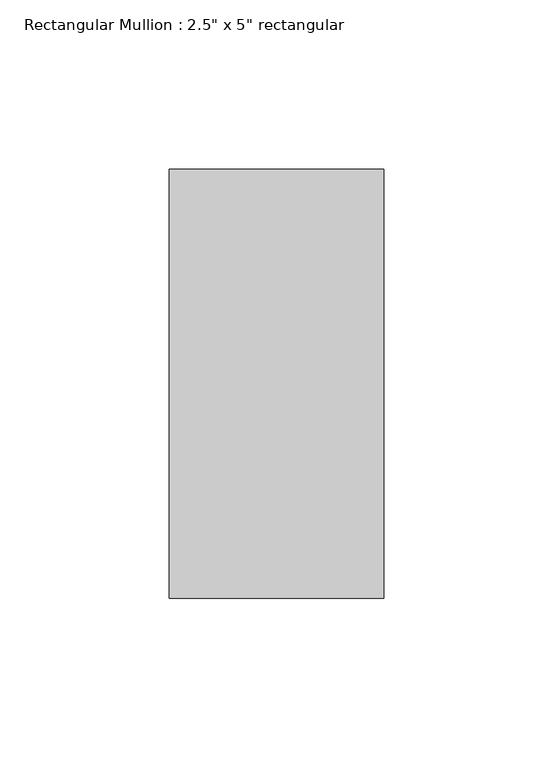
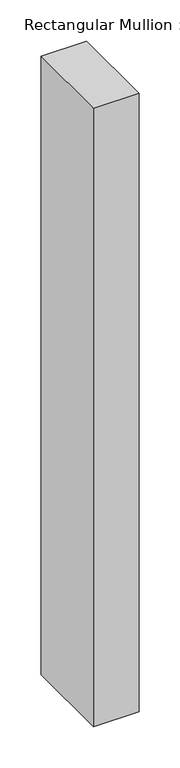
"""IFC4 building model written with IfcOpenShell, lengths in millimetres: member geometry."""

import ifcopenshell
import ifcopenshell.guid

model = None  # the IFC model being written
_history = None  # IfcOwnerHistory: only IFC2X3 demands one
_inside = {}  # id of a spatial element -> (the spatial element, [elements in it])
_under = {}  # id of a project, library or spatial element -> (it, [spatial elements below it])
_declared = {}  # id of a project -> (the project, [libraries it declares])
_typed = {}  # id of a type object -> (the type object, [elements of that type])
_made_of = {}  # id of a material, layer set ... -> (it, [elements and type objects made of it])


def new_model(schema):
    """Start an empty IFC model of exactly this schema.

    Asked for "IFC4X3", IfcOpenShell would pick the latest addendum, in which some entities
    have other attributes; the version numbers below select the first issue.
    IFC2X3 requires an IfcOwnerHistory on every rooted entity: one is made here for all.
    """
    global model, _history
    if schema == "IFC4X3":
        model = ifcopenshell.file(schema_version=(4, 3, 0, 0))
    else:
        model = ifcopenshell.file(schema=schema)
    _inside.clear()
    _under.clear()
    _declared.clear()
    _typed.clear()
    _made_of.clear()
    _history = None
    if model.schema == "IFC2X3":
        org = make("IfcOrganization", Name="unknown")
        user = make(
            "IfcPersonAndOrganization",
            ThePerson=make("IfcPerson", FamilyName="unknown"),
            TheOrganization=org,
        )
        app = make(
            "IfcApplication",
            ApplicationDeveloper=org,
            Version="unknown",
            ApplicationFullName="unknown",
            ApplicationIdentifier="unknown",
        )
        _history = make(
            "IfcOwnerHistory",
            OwningUser=user,
            OwningApplication=app,
            ChangeAction="ADDED",
            CreationDate=0,
        )
    return model


def make(cls, **values):
    """One entity of the class cls with the attributes given. An attribute that is None is left unset."""
    return model.create_entity(
        cls, **{name: value for name, value in values.items() if value is not None}
    )


def rooted(cls, **values):
    """An entity with a GlobalId (a new one), such as an element, a storey or a relation."""
    return make(cls, GlobalId=ifcopenshell.guid.new(), OwnerHistory=_history, **values)


def si_unit(unit_type, name, prefix=None):
    """IfcSIUnit, for example si_unit("LENGTHUNIT", "METRE", prefix="MILLI")."""
    return make("IfcSIUnit", UnitType=unit_type, Prefix=prefix, Name=name)


def assignment(units):
    """IfcUnitAssignment: the units of a project."""
    return None if units is None else make("IfcUnitAssignment", Units=units)


def point(xyz):
    """IfcCartesianPoint."""
    return None if xyz is None else make("IfcCartesianPoint", Coordinates=xyz)


def direction(xyz):
    """IfcDirection."""
    return None if xyz is None else make("IfcDirection", DirectionRatios=xyz)


def frame(location, z_axis=None, x_axis=None):
    """IfcAxis2Placement3D, a coordinate frame: its origin and axes. An axis left out is left unset."""
    return make(
        "IfcAxis2Placement3D",
        Location=point(location),
        Axis=direction(z_axis),
        RefDirection=direction(x_axis),
    )


def origin():
    """The frame at (0, 0, 0) with its axes left unset."""
    return frame((0.0, 0.0, 0.0))


def place(relative_to, where):
    """IfcLocalPlacement: puts the frame where relative to a parent placement (None: the world)."""
    return make(
        "IfcLocalPlacement", PlacementRelTo=relative_to, RelativePlacement=where
    )


def context(
    kind, dimensions, precision=None, world=None, true_north=None, identifier=None
):
    """IfcGeometricRepresentationContext, for example the 3D "Model" context."""
    return make(
        "IfcGeometricRepresentationContext",
        ContextIdentifier=identifier,
        ContextType=kind,
        CoordinateSpaceDimension=dimensions,
        Precision=precision,
        WorldCoordinateSystem=world,
        TrueNorth=true_north,
    )


def project(units=None, contexts=None):
    """IfcProject with its units and contexts."""
    return rooted(
        "IfcProject",
        Name="project",
        RepresentationContexts=contexts,
        UnitsInContext=assignment(units),
    )


def spatial(cls, under=None, at=None, **own):
    """A site, building, storey or space (cls), placed at a placement, below another one or the project."""
    s = rooted(cls, ObjectPlacement=at, **own)
    if under is not None:
        _under.setdefault(under.id(), (under, []))[1].append(s)
    return s


def polyline(points):
    """IfcPolyline through the points."""
    return make("IfcPolyline", Points=[point(p) for p in points])


def outline(outer, holes=None, kind="AREA"):
    """IfcArbitraryClosedProfileDef: a profile drawn as a closed curve; with holes, ...WithVoids."""
    if holes is None:
        return make("IfcArbitraryClosedProfileDef", ProfileType=kind, OuterCurve=outer)
    return make(
        "IfcArbitraryProfileDefWithVoids",
        ProfileType=kind,
        OuterCurve=outer,
        InnerCurves=holes,
    )


def extrude(swept, where, along, depth):
    """IfcExtrudedAreaSolid: the profile swept, set in the frame where, extruded along a direction by depth."""
    return make(
        "IfcExtrudedAreaSolid",
        SweptArea=swept,
        Position=where,
        ExtrudedDirection=direction(along),
        Depth=depth,
    )


def shape(context_of_items, identifier, shape_type, items):
    """IfcShapeRepresentation: the items that make up one representation, for example the "Body"."""
    return make(
        "IfcShapeRepresentation",
        ContextOfItems=context_of_items,
        RepresentationIdentifier=identifier,
        RepresentationType=shape_type,
        Items=items,
    )


def source(mapping_origin, context_of_items, identifier, shape_type, items):
    """IfcRepresentationMap: a shape defined once, which mapped items show again and again."""
    return make(
        "IfcRepresentationMap",
        MappingOrigin=mapping_origin,
        MappedRepresentation=shape(context_of_items, identifier, shape_type, items),
    )


def transform(
    local_origin,
    x_axis=None,
    y_axis=None,
    z_axis=None,
    scale=None,
    scale2=None,
    scale3=None,
    uniform=True,
):
    """IfcCartesianTransformationOperator3D, or its non-uniform kind. x_axis, y_axis, z_axis: its Axis1, 2, 3."""
    if uniform:
        return make(
            "IfcCartesianTransformationOperator3D",
            Axis1=direction(x_axis),
            Axis2=direction(y_axis),
            LocalOrigin=point(local_origin),
            Scale=scale,
            Axis3=direction(z_axis),
        )
    return make(
        "IfcCartesianTransformationOperator3DnonUniform",
        Axis1=direction(x_axis),
        Axis2=direction(y_axis),
        LocalOrigin=point(local_origin),
        Scale=scale,
        Axis3=direction(z_axis),
        Scale2=scale2,
        Scale3=scale3,
    )


def mapped(mapping_source, mapping_target):
    """IfcMappedItem: shows the shape of a source again, moved by a transform."""
    return make(
        "IfcMappedItem", MappingSource=mapping_source, MappingTarget=mapping_target
    )


def made_of(thing, what):
    """Note that an element or type object is made of a material, layer set ...; save() writes the relation."""
    if what is not None:
        _made_of.setdefault(what.id(), (what, []))[1].append(thing)
    return thing


def element(
    cls,
    number,
    at=None,
    inside=None,
    cuts=None,
    type_object=None,
    material=None,
    context=None,
    identifier="Body",
    shape_type=None,
    held_by="IfcProductDefinitionShape",
    body=None,
    shapes=None,
    **own,
):
    """One element of the class cls, such as IfcWall. Its Tag is "e" and its number.

    at: its placement. inside: the storey or other place that contains it. cuts: it is an
    opening in that element (IfcRelVoidsElement). A single representation is given by context,
    identifier, shape_type and body (its items); several are given by shapes. held_by: the class
    of the entity that holds the representations. save() writes the other relations.
    """
    e = rooted(cls, Tag="e%d" % number, ObjectPlacement=at, **own)
    if body is not None:
        shapes = [shape(context, identifier, shape_type, body)]
    if shapes is not None:
        e.Representation = make(held_by, Representations=shapes)
    if inside is not None:
        _inside.setdefault(inside.id(), (inside, []))[1].append(e)
    if cuts is not None:
        rooted(
            "IfcRelVoidsElement", RelatingBuildingElement=cuts, RelatedOpeningElement=e
        )
    if type_object is not None:
        _typed.setdefault(type_object.id(), (type_object, []))[1].append(e)
    return made_of(e, material)


def aggregate(whole, parts):
    """IfcRelAggregates: a whole, such as a stair, and the parts it consists of."""
    return rooted("IfcRelAggregates", RelatingObject=whole, RelatedObjects=parts)


def save(model, path):
    """Write the relations noted so far, then the file.

    IfcRelAggregates (storeys below a building ...), IfcRelContainedInSpatialStructure (elements
    in a storey), IfcRelDefinesByType, IfcRelAssociatesMaterial and IfcRelDeclares: one each for
    every whole, place, type object, material and project.
    """
    for whole, parts in _under.values():
        aggregate(whole, parts)
    for where, things in _inside.values():
        rooted(
            "IfcRelContainedInSpatialStructure",
            RelatedElements=things,
            RelatingStructure=where,
        )
    for kind, things in _typed.values():
        rooted("IfcRelDefinesByType", RelatedObjects=things, RelatingType=kind)
    for what, things in _made_of.values():
        rooted("IfcRelAssociatesMaterial", RelatedObjects=things, RelatingMaterial=what)
    for by, libraries in _declared.values():
        rooted("IfcRelDeclares", RelatingContext=by, RelatedDefinitions=libraries)
    model.write(path)


def member_410c6227(model_context):
    return source(origin(), model_context, "Body", "SweptSolid", [
        extrude(outline(polyline([(31.75, 63.5), (31.75, -63.5), (-31.75, -63.5), (-31.75, 63.5), (31.75, 63.5)])), frame((0.0, 0.0, -914.4), z_axis=(0.0, 0.0, 1.0), x_axis=(1.0, 0.0, 0.0)), (0.0, 0.0, 1.0), 914.4),
    ])


if __name__ == "__main__":
    model = new_model("IFC4")
    model_context = context("Model", 3, world=origin())
    ifc_project = project(units=[si_unit("LENGTHUNIT", "METRE", prefix="MILLI")], contexts=[model_context])
    site = spatial("IfcSite", under=ifc_project)
    building = spatial("IfcBuilding", under=site)
    placement = place(None, origin())
    member_shape = member_410c6227(model_context)
    element("IfcMember", 1, ObjectType="Rectangular Mullion : 2.5\" x 5\" rectangular", at=placement, inside=building, context=model_context, shape_type="MappedRepresentation", body=[
        mapped(member_shape, transform((0.0, 0.0, 0.0), x_axis=(1.0, 0.0, 0.0), y_axis=(0.0, 1.0, 0.0), z_axis=(0.0, 0.0, 1.0))),
    ])
    save(model, "model.ifc")

# Revit data of these elements
# Type "Rectangular Mullion : 2.5\" x 5\" rectangular"
#   built-in parameter 1007304 = 0.416667 (stored number, unit not read)
#   built-in parameter 1007301 = 0.104167 (stored number, unit not read)
#   built-in parameter 1007300 = 0.104167 (stored number, unit not read)
# Element 1 (IfcMember, "Rectangular Mullion : 2.5\" x 5\" rectangular")
#   Materials on its faces: "Aluminum"
# Materials
#   "Aluminum": class "Metal", colour RGB 247 247 247, transparency 0, Description = "Aluminum 6061", Cost = 0
